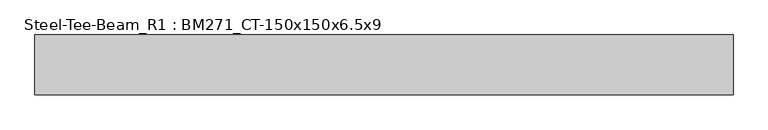
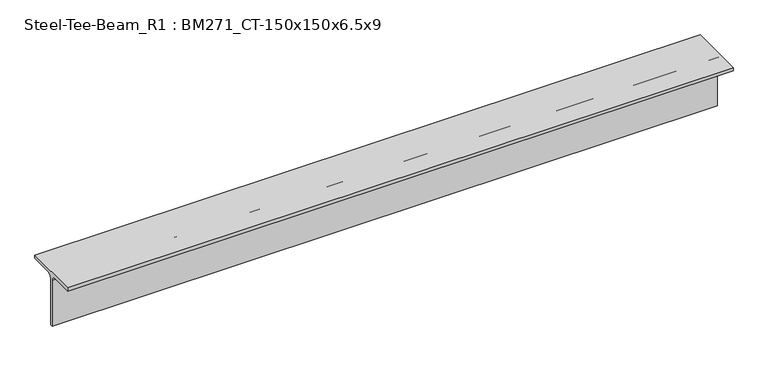
"""IFC4 building model written with IfcOpenShell, lengths in millimetres: member geometry, Steel-Tee-Beam_R1 : BM271_CT-150x150x6.5x9."""

from ifc_helpers import new_model, si_unit, point, frame, frame_2d, origin, place, context, project, spatial, polyline, circle_curve, trimmed, segment, composite_curve, outline, extrude, source, transform, mapped, element, save


def steel_tee_beam_r1_bm271_ct_150x150x6_5x9_172c8867(model_context):
    return source(origin(), model_context, "Body", "SweptSolid", [
        extrude(outline(composite_curve([segment(polyline([(-75.0, 75.0), (75.0, 75.0), (75.0, 66.0), (16.25, 66.0)]), True, "CONTINUOUS"), segment(trimmed(circle_curve(frame_2d((16.25, 53.0)), 13.0), [point((16.25, 66.0))], [point((3.25, 53.0))], True, "CARTESIAN"), True, "CONTINUOUS"), segment(polyline([(3.25, 53.0), (3.25, -75.0), (-3.25, -75.0), (-3.25, 53.0)]), True, "CONTINUOUS"), segment(trimmed(circle_curve(frame_2d((-16.25, 53.0)), 13.0), [point((-3.25, 53.0))], [point((-16.25, 66.0))], True, "CARTESIAN"), True, "CONTINUOUS"), segment(polyline([(-16.25, 66.0), (-75.0, 66.0), (-75.0, 75.0)]), True, "CONTINUOUS")], self_intersect=False)), frame((-770.8583806, 0.0, 0.0), z_axis=(1.0, 0.0, 0.0), x_axis=(0.0, 1.0, 0.0)), (0.0, 0.0, 1.0), 1754.8398202),
    ])


if __name__ == "__main__":
    model = new_model("IFC4")
    model_context = context("Model", 3, world=origin())
    ifc_project = project(units=[si_unit("LENGTHUNIT", "METRE", prefix="MILLI")], contexts=[model_context])
    site = spatial("IfcSite", under=ifc_project)
    building = spatial("IfcBuilding", under=site)
    placement = place(None, origin())
    steel_tee_beam_r1_bm271_ct_150x150x6_5x9_shape = steel_tee_beam_r1_bm271_ct_150x150x6_5x9_172c8867(model_context)
    element("IfcMember", 1, ObjectType="Steel-Tee-Beam_R1 : BM271_CT-150x150x6.5x9", at=placement, inside=building, context=model_context, shape_type="MappedRepresentation", body=[
        mapped(steel_tee_beam_r1_bm271_ct_150x150x6_5x9_shape, transform((0.0, 0.0, 0.0), x_axis=(1.0, 0.0, 0.0), y_axis=(0.0, 1.0, 0.0), z_axis=(0.0, 0.0, 1.0))),
    ])
    save(model, "model.ifc")

# Revit data of these elements
# Type "Steel-Tee-Beam_R1 : BM271_CT-150x150x6.5x9"
#   Keynote = "CT-150x150x6.5x9"
#   Surface Area = 0.588841 m²/m
#   Section Area = 23.3904 cm²
#   Mass per Unit Length = 18.3614 kg/m
#   Length [instance default] = 1.5240 m
#   bf = 0.1500 m
#   d = 0.1500 m
#   k = 0.0220 m
#   r = 0.0130 m
#   tf = 0.0090 m
#   tw = 0.0065 m
#   hec_material4 [instance default] = none
#   hec_material3 [instance default] = none
#   hec_material2 [instance default] = none
#   hec_material1 [instance default] = none
#   Structural Material [instance default] = Steel, 45-345
#   Assembly Code = ""
# Element 1 (IfcMember, "Steel-Tee-Beam_R1 : BM271_CT-150x150x6.5x9")
#   Structural Material = none
# Materials
#   "Steel, 45-345": class "Metal", colour RGB 189 187 185, transparency 0, Description = "Steel 345 MPa", Cost = 0
